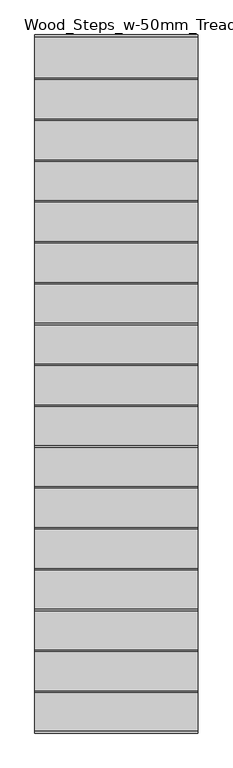
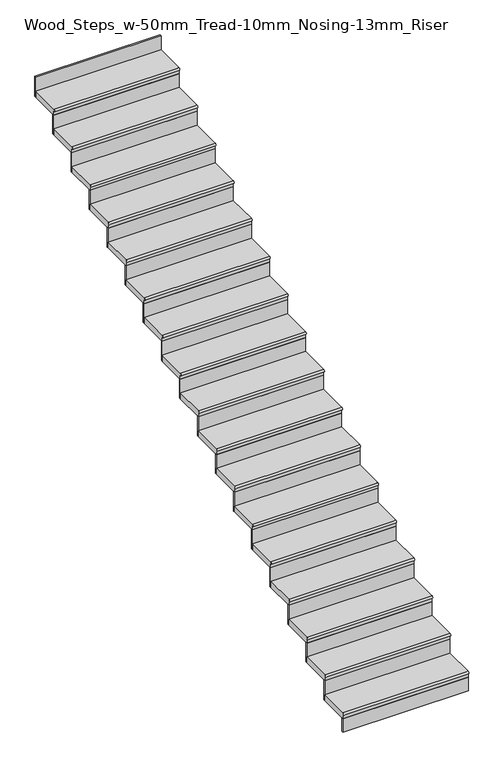
"""IFC4 building model written with IfcOpenShell, lengths in millimetres: stair flight geometry, Wood_Steps_w-50mm_Tread-10mm_Nosing-13mm_Riser."""

from ifc_helpers import new_model, si_unit, point, frame, frame_2d, origin, origin_with_axes, place, context, project, spatial, polyline, circle_curve, trimmed, segment, composite_curve, outline, extrude, source, transform, mapped, element, save


def wood_steps_w_50mm_tread_10mm_nosing_13mm_riser_9048c9ab(model_context):
    return source(origin(), model_context, "Body", "SweptSolid", [
        extrude(outline(composite_curve([segment(polyline([(-4299.5613451, 166.6666667), (-4049.5613451, 166.6666667), (-4049.5613451, 116.6666667), (-4299.5613451, 116.6666667), (-4299.5613451, 146.6666667)]), True, "CONTINUOUS"), segment(trimmed(circle_curve(frame_2d((-4299.5613451, 156.6666667)), 10.0), [point((-4299.5613451, 146.6666667))], [point((-4299.5613451, 166.6666667))], False, "CARTESIAN"), True, "CONTINUOUS")], self_intersect=False)), frame((2159.5846643, 0.0, 0.0), z_axis=(1.0, 0.0, 0.0), x_axis=(0.0, 1.0, 0.0)), (0.0, 0.0, 1.0), 1000.0),
        extrude(outline(polyline([(3159.5846643, -4287.0613451), (3159.5846643, -4299.5613451), (2159.5846643, -4299.5613451), (2159.5846643, -4287.0613451), (3159.5846643, -4287.0613451)])), origin_with_axes(), (0.0, 0.0, 1.0), 116.6666667),
        extrude(outline(polyline([(3159.5846643, -4037.0613451), (3159.5846643, -4049.5613451), (2159.5846643, -4049.5613451), (2159.5846643, -4037.0613451), (3159.5846643, -4037.0613451)])), frame((0.0, 0.0, 116.6666667), z_axis=(0.0, 0.0, 1.0), x_axis=(1.0, 0.0, 0.0)), (0.0, 0.0, 1.0), 166.6666667),
        extrude(outline(composite_curve([segment(polyline([(-4049.5613451, 333.3333333), (-3799.5613451, 333.3333333), (-3799.5613451, 283.3333333), (-4049.5613451, 283.3333333), (-4049.5613451, 313.3333333)]), True, "CONTINUOUS"), segment(trimmed(circle_curve(frame_2d((-4049.5613451, 323.3333333)), 10.0), [point((-4049.5613451, 313.3333333))], [point((-4049.5613451, 333.3333333))], False, "CARTESIAN"), True, "CONTINUOUS")], self_intersect=False)), frame((2159.5846643, 0.0, 0.0), z_axis=(1.0, 0.0, 0.0), x_axis=(0.0, 1.0, 0.0)), (0.0, 0.0, 1.0), 1000.0),
        extrude(outline(polyline([(3159.5846643, -3787.0613451), (3159.5846643, -3799.5613451), (2159.5846643, -3799.5613451), (2159.5846643, -3787.0613451), (3159.5846643, -3787.0613451)])), frame((0.0, 0.0, 283.3333333), z_axis=(0.0, 0.0, 1.0), x_axis=(1.0, 0.0, 0.0)), (0.0, 0.0, 1.0), 166.6666667),
        extrude(outline(composite_curve([segment(polyline([(-3799.5613451, 500.0), (-3549.5613451, 500.0), (-3549.5613451, 450.0), (-3799.5613451, 450.0), (-3799.5613451, 480.0)]), True, "CONTINUOUS"), segment(trimmed(circle_curve(frame_2d((-3799.5613451, 490.0)), 10.0), [point((-3799.5613451, 480.0))], [point((-3799.5613451, 500.0))], False, "CARTESIAN"), True, "CONTINUOUS")], self_intersect=False)), frame((2159.5846643, 0.0, 0.0), z_axis=(1.0, 0.0, 0.0), x_axis=(0.0, 1.0, 0.0)), (0.0, 0.0, 1.0), 1000.0),
        extrude(outline(polyline([(3159.5846643, -3537.0613451), (3159.5846643, -3549.5613451), (2159.5846643, -3549.5613451), (2159.5846643, -3537.0613451), (3159.5846643, -3537.0613451)])), frame((0.0, 0.0, 450.0), z_axis=(0.0, 0.0, 1.0), x_axis=(1.0, 0.0, 0.0)), (0.0, 0.0, 1.0), 166.6666667),
        extrude(outline(composite_curve([segment(polyline([(-3549.5613451, 666.6666667), (-3299.5613451, 666.6666667), (-3299.5613451, 616.6666667), (-3549.5613451, 616.6666667), (-3549.5613451, 646.6666667)]), True, "CONTINUOUS"), segment(trimmed(circle_curve(frame_2d((-3549.5613451, 656.6666667)), 10.0), [point((-3549.5613451, 646.6666667))], [point((-3549.5613451, 666.6666667))], False, "CARTESIAN"), True, "CONTINUOUS")], self_intersect=False)), frame((2159.5846643, 0.0, 0.0), z_axis=(1.0, 0.0, 0.0), x_axis=(0.0, 1.0, 0.0)), (0.0, 0.0, 1.0), 1000.0),
        extrude(outline(polyline([(3159.5846643, -3287.0613451), (3159.5846643, -3299.5613451), (2159.5846643, -3299.5613451), (2159.5846643, -3287.0613451), (3159.5846643, -3287.0613451)])), frame((0.0, 0.0, 616.6666667), z_axis=(0.0, 0.0, 1.0), x_axis=(1.0, 0.0, 0.0)), (0.0, 0.0, 1.0), 166.6666667),
        extrude(outline(composite_curve([segment(polyline([(-3299.5613451, 833.3333333), (-3049.5613451, 833.3333333), (-3049.5613451, 783.3333333), (-3299.5613451, 783.3333333), (-3299.5613451, 813.3333333)]), True, "CONTINUOUS"), segment(trimmed(circle_curve(frame_2d((-3299.5613451, 823.3333333)), 10.0), [point((-3299.5613451, 813.3333333))], [point((-3299.5613451, 833.3333333))], False, "CARTESIAN"), True, "CONTINUOUS")], self_intersect=False)), frame((2159.5846643, 0.0, 0.0), z_axis=(1.0, 0.0, 0.0), x_axis=(0.0, 1.0, 0.0)), (0.0, 0.0, 1.0), 1000.0),
        extrude(outline(polyline([(3159.5846643, -3037.0613451), (3159.5846643, -3049.5613451), (2159.5846643, -3049.5613451), (2159.5846643, -3037.0613451), (3159.5846643, -3037.0613451)])), frame((0.0, 0.0, 783.3333333), z_axis=(0.0, 0.0, 1.0), x_axis=(1.0, 0.0, 0.0)), (0.0, 0.0, 1.0), 166.6666667),
        extrude(outline(composite_curve([segment(polyline([(-3049.5613451, 1000.0), (-2799.5613451, 1000.0), (-2799.5613451, 950.0), (-3049.5613451, 950.0), (-3049.5613451, 980.0)]), True, "CONTINUOUS"), segment(trimmed(circle_curve(frame_2d((-3049.5613451, 990.0)), 10.0), [point((-3049.5613451, 980.0))], [point((-3049.5613451, 1000.0))], False, "CARTESIAN"), True, "CONTINUOUS")], self_intersect=False)), frame((2159.5846643, 0.0, 0.0), z_axis=(1.0, 0.0, 0.0), x_axis=(0.0, 1.0, 0.0)), (0.0, 0.0, 1.0), 1000.0),
        extrude(outline(polyline([(3159.5846643, -2787.0613451), (3159.5846643, -2799.5613451), (2159.5846643, -2799.5613451), (2159.5846643, -2787.0613451), (3159.5846643, -2787.0613451)])), frame((0.0, 0.0, 950.0), z_axis=(0.0, 0.0, 1.0), x_axis=(1.0, 0.0, 0.0)), (0.0, 0.0, 1.0), 166.6666667),
        extrude(outline(composite_curve([segment(polyline([(-2799.5613451, 1166.6666667), (-2549.5613451, 1166.6666667), (-2549.5613451, 1116.6666667), (-2799.5613451, 1116.6666667), (-2799.5613451, 1146.6666667)]), True, "CONTINUOUS"), segment(trimmed(circle_curve(frame_2d((-2799.5613451, 1156.6666667)), 10.0), [point((-2799.5613451, 1146.6666667))], [point((-2799.5613451, 1166.6666667))], False, "CARTESIAN"), True, "CONTINUOUS")], self_intersect=False)), frame((2159.5846643, 0.0, 0.0), z_axis=(1.0, 0.0, 0.0), x_axis=(0.0, 1.0, 0.0)), (0.0, 0.0, 1.0), 1000.0),
        extrude(outline(polyline([(3159.5846643, -2537.0613451), (3159.5846643, -2549.5613451), (2159.5846643, -2549.5613451), (2159.5846643, -2537.0613451), (3159.5846643, -2537.0613451)])), frame((0.0, 0.0, 1116.6666667), z_axis=(0.0, 0.0, 1.0), x_axis=(1.0, 0.0, 0.0)), (0.0, 0.0, 1.0), 166.6666667),
        extrude(outline(composite_curve([segment(polyline([(-2549.5613451, 1333.3333333), (-2299.5613451, 1333.3333333), (-2299.5613451, 1283.3333333), (-2549.5613451, 1283.3333333), (-2549.5613451, 1313.3333333)]), True, "CONTINUOUS"), segment(trimmed(circle_curve(frame_2d((-2549.5613451, 1323.3333333)), 10.0), [point((-2549.5613451, 1313.3333333))], [point((-2549.5613451, 1333.3333333))], False, "CARTESIAN"), True, "CONTINUOUS")], self_intersect=False)), frame((2159.5846643, 0.0, 0.0), z_axis=(1.0, 0.0, 0.0), x_axis=(0.0, 1.0, 0.0)), (0.0, 0.0, 1.0), 1000.0),
        extrude(outline(polyline([(3159.5846643, -2287.0613451), (3159.5846643, -2299.5613451), (2159.5846643, -2299.5613451), (2159.5846643, -2287.0613451), (3159.5846643, -2287.0613451)])), frame((0.0, 0.0, 1283.3333333), z_axis=(0.0, 0.0, 1.0), x_axis=(1.0, 0.0, 0.0)), (0.0, 0.0, 1.0), 166.6666667),
        extrude(outline(composite_curve([segment(polyline([(-2299.5613451, 1500.0), (-2049.5613451, 1500.0), (-2049.5613451, 1450.0), (-2299.5613451, 1450.0), (-2299.5613451, 1480.0)]), True, "CONTINUOUS"), segment(trimmed(circle_curve(frame_2d((-2299.5613451, 1490.0)), 10.0), [point((-2299.5613451, 1480.0))], [point((-2299.5613451, 1500.0))], False, "CARTESIAN"), True, "CONTINUOUS")], self_intersect=False)), frame((2159.5846643, 0.0, 0.0), z_axis=(1.0, 0.0, 0.0), x_axis=(0.0, 1.0, 0.0)), (0.0, 0.0, 1.0), 1000.0),
        extrude(outline(polyline([(3159.5846643, -2037.0613451), (3159.5846643, -2049.5613451), (2159.5846643, -2049.5613451), (2159.5846643, -2037.0613451), (3159.5846643, -2037.0613451)])), frame((0.0, 0.0, 1450.0), z_axis=(0.0, 0.0, 1.0), x_axis=(1.0, 0.0, 0.0)), (0.0, 0.0, 1.0), 166.6666667),
        extrude(outline(composite_curve([segment(polyline([(-2049.5613451, 1666.6666667), (-1799.5613451, 1666.6666667), (-1799.5613451, 1616.6666667), (-2049.5613451, 1616.6666667), (-2049.5613451, 1646.6666667)]), True, "CONTINUOUS"), segment(trimmed(circle_curve(frame_2d((-2049.5613451, 1656.6666667)), 10.0), [point((-2049.5613451, 1646.6666667))], [point((-2049.5613451, 1666.6666667))], False, "CARTESIAN"), True, "CONTINUOUS")], self_intersect=False)), frame((2159.5846643, 0.0, 0.0), z_axis=(1.0, 0.0, 0.0), x_axis=(0.0, 1.0, 0.0)), (0.0, 0.0, 1.0), 1000.0),
        extrude(outline(polyline([(3159.5846643, -1787.0613451), (3159.5846643, -1799.5613451), (2159.5846643, -1799.5613451), (2159.5846643, -1787.0613451), (3159.5846643, -1787.0613451)])), frame((0.0, 0.0, 1616.6666667), z_axis=(0.0, 0.0, 1.0), x_axis=(1.0, 0.0, 0.0)), (0.0, 0.0, 1.0), 166.6666667),
        extrude(outline(composite_curve([segment(polyline([(-1799.5613451, 1833.3333333), (-1549.5613451, 1833.3333333), (-1549.5613451, 1783.3333333), (-1799.5613451, 1783.3333333), (-1799.5613451, 1813.3333333)]), True, "CONTINUOUS"), segment(trimmed(circle_curve(frame_2d((-1799.5613451, 1823.3333333)), 10.0), [point((-1799.5613451, 1813.3333333))], [point((-1799.5613451, 1833.3333333))], False, "CARTESIAN"), True, "CONTINUOUS")], self_intersect=False)), frame((2159.5846643, 0.0, 0.0), z_axis=(1.0, 0.0, 0.0), x_axis=(0.0, 1.0, 0.0)), (0.0, 0.0, 1.0), 1000.0),
        extrude(outline(polyline([(3159.5846643, -1537.0613451), (3159.5846643, -1549.5613451), (2159.5846643, -1549.5613451), (2159.5846643, -1537.0613451), (3159.5846643, -1537.0613451)])), frame((0.0, 0.0, 1783.3333333), z_axis=(0.0, 0.0, 1.0), x_axis=(1.0, 0.0, 0.0)), (0.0, 0.0, 1.0), 166.6666667),
        extrude(outline(composite_curve([segment(polyline([(-1549.5613451, 2000.0), (-1299.5613451, 2000.0), (-1299.5613451, 1950.0), (-1549.5613451, 1950.0), (-1549.5613451, 1980.0)]), True, "CONTINUOUS"), segment(trimmed(circle_curve(frame_2d((-1549.5613451, 1990.0)), 10.0), [point((-1549.5613451, 1980.0))], [point((-1549.5613451, 2000.0))], False, "CARTESIAN"), True, "CONTINUOUS")], self_intersect=False)), frame((2159.5846643, 0.0, 0.0), z_axis=(1.0, 0.0, 0.0), x_axis=(0.0, 1.0, 0.0)), (0.0, 0.0, 1.0), 1000.0),
        extrude(outline(polyline([(3159.5846643, -1287.0613451), (3159.5846643, -1299.5613451), (2159.5846643, -1299.5613451), (2159.5846643, -1287.0613451), (3159.5846643, -1287.0613451)])), frame((0.0, 0.0, 1950.0), z_axis=(0.0, 0.0, 1.0), x_axis=(1.0, 0.0, 0.0)), (0.0, 0.0, 1.0), 166.6666667),
        extrude(outline(composite_curve([segment(polyline([(-1299.5613451, 2166.6666667), (-1049.5613451, 2166.6666667), (-1049.5613451, 2116.6666667), (-1299.5613451, 2116.6666667), (-1299.5613451, 2146.6666667)]), True, "CONTINUOUS"), segment(trimmed(circle_curve(frame_2d((-1299.5613451, 2156.6666667)), 10.0), [point((-1299.5613451, 2146.6666667))], [point((-1299.5613451, 2166.6666667))], False, "CARTESIAN"), True, "CONTINUOUS")], self_intersect=False)), frame((2159.5846643, 0.0, 0.0), z_axis=(1.0, 0.0, 0.0), x_axis=(0.0, 1.0, 0.0)), (0.0, 0.0, 1.0), 1000.0),
        extrude(outline(polyline([(3159.5846643, -1037.0613451), (3159.5846643, -1049.5613451), (2159.5846643, -1049.5613451), (2159.5846643, -1037.0613451), (3159.5846643, -1037.0613451)])), frame((0.0, 0.0, 2116.6666667), z_axis=(0.0, 0.0, 1.0), x_axis=(1.0, 0.0, 0.0)), (0.0, 0.0, 1.0), 166.6666667),
        extrude(outline(composite_curve([segment(polyline([(-1049.5613451, 2333.3333333), (-799.5613451, 2333.3333333), (-799.5613451, 2283.3333333), (-1049.5613451, 2283.3333333), (-1049.5613451, 2313.3333333)]), True, "CONTINUOUS"), segment(trimmed(circle_curve(frame_2d((-1049.5613451, 2323.3333333)), 10.0), [point((-1049.5613451, 2313.3333333))], [point((-1049.5613451, 2333.3333333))], False, "CARTESIAN"), True, "CONTINUOUS")], self_intersect=False)), frame((2159.5846643, 0.0, 0.0), z_axis=(1.0, 0.0, 0.0), x_axis=(0.0, 1.0, 0.0)), (0.0, 0.0, 1.0), 1000.0),
        extrude(outline(polyline([(3159.5846643, -787.0613451), (3159.5846643, -799.5613451), (2159.5846643, -799.5613451), (2159.5846643, -787.0613451), (3159.5846643, -787.0613451)])), frame((0.0, 0.0, 2283.3333333), z_axis=(0.0, 0.0, 1.0), x_axis=(1.0, 0.0, 0.0)), (0.0, 0.0, 1.0), 166.6666667),
        extrude(outline(composite_curve([segment(polyline([(-799.5613451, 2500.0), (-549.5613451, 2500.0), (-549.5613451, 2450.0), (-799.5613451, 2450.0), (-799.5613451, 2480.0)]), True, "CONTINUOUS"), segment(trimmed(circle_curve(frame_2d((-799.5613451, 2490.0)), 10.0), [point((-799.5613451, 2480.0))], [point((-799.5613451, 2500.0))], False, "CARTESIAN"), True, "CONTINUOUS")], self_intersect=False)), frame((2159.5846643, 0.0, 0.0), z_axis=(1.0, 0.0, 0.0), x_axis=(0.0, 1.0, 0.0)), (0.0, 0.0, 1.0), 1000.0),
        extrude(outline(polyline([(3159.5846643, -537.0613451), (3159.5846643, -549.5613451), (2159.5846643, -549.5613451), (2159.5846643, -537.0613451), (3159.5846643, -537.0613451)])), frame((0.0, 0.0, 2450.0), z_axis=(0.0, 0.0, 1.0), x_axis=(1.0, 0.0, 0.0)), (0.0, 0.0, 1.0), 166.6666667),
        extrude(outline(composite_curve([segment(polyline([(-549.5613451, 2666.6666667), (-299.5613451, 2666.6666667), (-299.5613451, 2616.6666667), (-549.5613451, 2616.6666667), (-549.5613451, 2646.6666667)]), True, "CONTINUOUS"), segment(trimmed(circle_curve(frame_2d((-549.5613451, 2656.6666667)), 10.0), [point((-549.5613451, 2646.6666667))], [point((-549.5613451, 2666.6666667))], False, "CARTESIAN"), True, "CONTINUOUS")], self_intersect=False)), frame((2159.5846643, 0.0, 0.0), z_axis=(1.0, 0.0, 0.0), x_axis=(0.0, 1.0, 0.0)), (0.0, 0.0, 1.0), 1000.0),
        extrude(outline(polyline([(3159.5846643, -287.0613451), (3159.5846643, -299.5613451), (2159.5846643, -299.5613451), (2159.5846643, -287.0613451), (3159.5846643, -287.0613451)])), frame((0.0, 0.0, 2616.6666667), z_axis=(0.0, 0.0, 1.0), x_axis=(1.0, 0.0, 0.0)), (0.0, 0.0, 1.0), 166.6666667),
        extrude(outline(polyline([(3159.5846643, -37.0613451), (3159.5846643, -49.5613451), (2159.5846643, -49.5613451), (2159.5846643, -37.0613451), (3159.5846643, -37.0613451)])), frame((0.0, 0.0, 2783.3333333), z_axis=(0.0, 0.0, 1.0), x_axis=(1.0, 0.0, 0.0)), (0.0, 0.0, 1.0), 166.6666667),
        extrude(outline(composite_curve([segment(polyline([(-299.5613451, 2833.3333333), (-49.5613451, 2833.3333333), (-49.5613451, 2783.3333333), (-299.5613451, 2783.3333333), (-299.5613451, 2813.3333333)]), True, "CONTINUOUS"), segment(trimmed(circle_curve(frame_2d((-299.5613451, 2823.3333333)), 10.0), [point((-299.5613451, 2813.3333333))], [point((-299.5613451, 2833.3333333))], False, "CARTESIAN"), True, "CONTINUOUS")], self_intersect=False)), frame((2159.5846643, 0.0, 0.0), z_axis=(1.0, 0.0, 0.0), x_axis=(0.0, 1.0, 0.0)), (0.0, 0.0, 1.0), 1000.0),
    ])


if __name__ == "__main__":
    model = new_model("IFC4")
    model_context = context("Model", 3, world=origin())
    ifc_project = project(units=[si_unit("LENGTHUNIT", "METRE", prefix="MILLI")], contexts=[model_context])
    site = spatial("IfcSite", under=ifc_project)
    building = spatial("IfcBuilding", under=site)
    placement = place(None, origin())
    wood_steps_w_50mm_tread_10mm_nosing_13mm_riser_shape = wood_steps_w_50mm_tread_10mm_nosing_13mm_riser_9048c9ab(model_context)
    element("IfcStairFlight", 1, ObjectType="Wood_Steps_w-50mm_Tread-10mm_Nosing-13mm_Riser", at=placement, inside=building, context=model_context, shape_type="MappedRepresentation", body=[
        mapped(wood_steps_w_50mm_tread_10mm_nosing_13mm_riser_shape, transform((0.0, 0.0, 0.0), x_axis=(1.0, 0.0, 0.0), y_axis=(0.0, 1.0, 0.0), z_axis=(0.0, 0.0, 1.0))),
    ])
    save(model, "model.ifc")

# Revit data of these elements
# Element 1 (IfcStairFlight, "Wood_Steps_w-50mm_Tread-10mm_Nosing-13mm_Riser")
#   Materials on its faces: "Oak Flooring"
# Materials
#   "Oak Flooring": class "Wood", colour RGB 212 179 113, transparency 0, Description = "Quercus Rubra", Cost = 0
